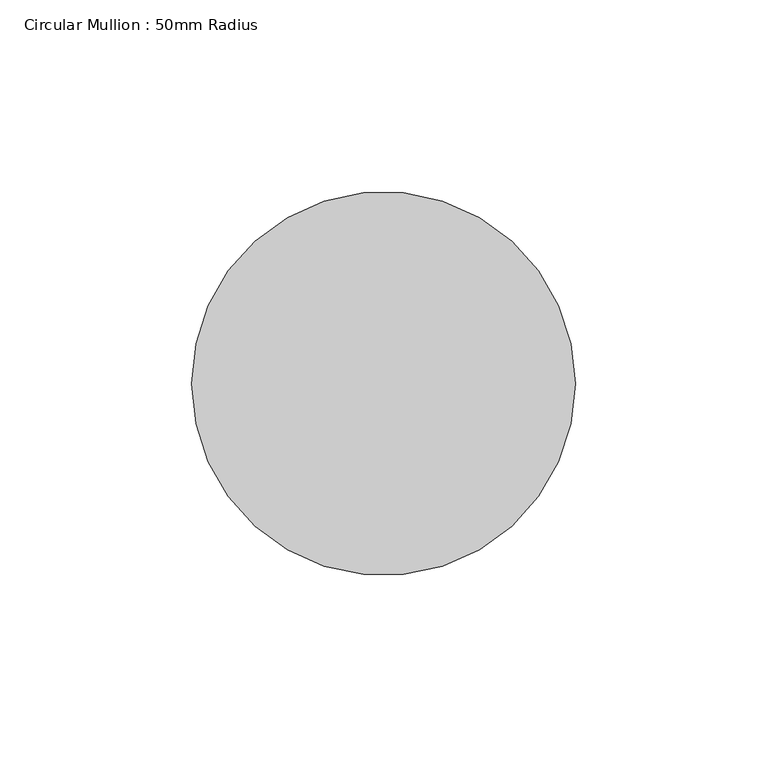
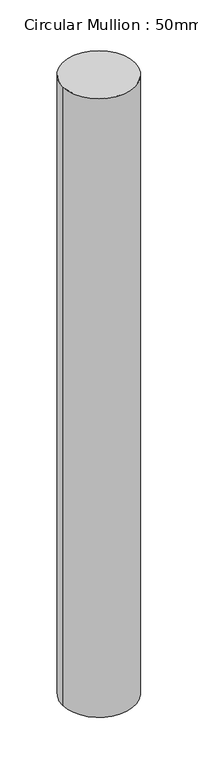
"""IFC4 building model written with IfcOpenShell, lengths in millimetres: member geometry, Circular Mullion : 50mm Radius."""

from ifc_helpers import new_model, si_unit, point, frame, origin, origin_2d, place, context, project, spatial, circle_curve, trimmed, segment, composite_curve, outline, extrude, source, transform, mapped, element, save


def circular_mullion_50mm_radius_828f0cec(model_context):
    return source(origin(), model_context, "Body", "SweptSolid", [
        extrude(outline(composite_curve([segment(trimmed(circle_curve(origin_2d(), 50.0), [point((50.0, 0.0))], [point((-50.0, 0.0))], False, "CARTESIAN"), True, "CONTINUOUS"), segment(trimmed(circle_curve(origin_2d(), 50.0), [point((-50.0, 0.0))], [point((50.0, 0.0))], False, "CARTESIAN"), True, "CONTINUOUS")], self_intersect=False)), frame((0.0, 0.0, -902.1263791), z_axis=(0.0, 0.0, 1.0), x_axis=(1.0, 0.0, 0.0)), (0.0, 0.0, 1.0), 902.1263791),
    ])


if __name__ == "__main__":
    model = new_model("IFC4")
    model_context = context("Model", 3, world=origin())
    ifc_project = project(units=[si_unit("LENGTHUNIT", "METRE", prefix="MILLI")], contexts=[model_context])
    site = spatial("IfcSite", under=ifc_project)
    building = spatial("IfcBuilding", under=site)
    placement = place(None, origin())
    circular_mullion_50mm_radius_shape = circular_mullion_50mm_radius_828f0cec(model_context)
    element("IfcMember", 1, ObjectType="Circular Mullion : 50mm Radius", at=placement, inside=building, context=model_context, shape_type="MappedRepresentation", body=[
        mapped(circular_mullion_50mm_radius_shape, transform((0.0, 0.0, 0.0), x_axis=(1.0, 0.0, 0.0), y_axis=(0.0, 1.0, 0.0), z_axis=(0.0, 0.0, 1.0))),
    ])
    save(model, "model.ifc")

# Revit data of these elements
# Type "Circular Mullion : 50mm Radius"
#   built-in parameter 1007350 = 0.164042 (stored number, unit not read)
# Element 1 (IfcMember, "Circular Mullion : 50mm Radius")
#   Materials on its faces: "Aluminium"
# Materials
#   "Aluminium": class "Metal", colour RGB 247 247 247, transparency 0, Description = "Aluminium 6061", Cost = 0
